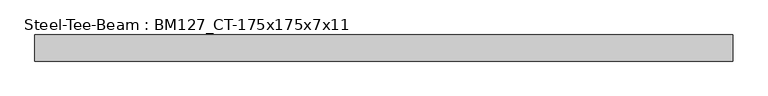
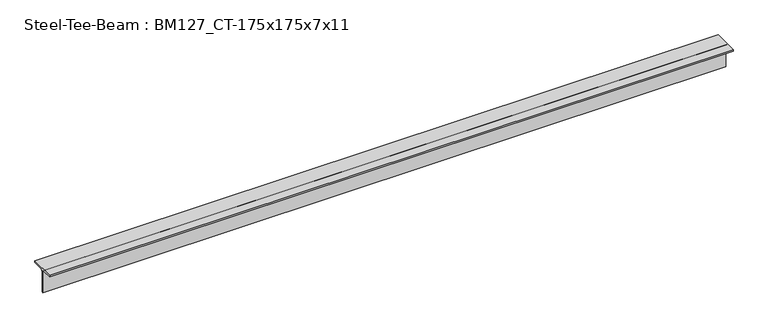
"""IFC4 building model written with IfcOpenShell, lengths in millimetres: beam geometry, Steel-Tee-Beam : BM127_CT-175x175x7x11."""

import ifcopenshell
import ifcopenshell.guid

model = None  # the IFC model being written
_history = None  # IfcOwnerHistory: only IFC2X3 demands one
_inside = {}  # id of a spatial element -> (the spatial element, [elements in it])
_under = {}  # id of a project, library or spatial element -> (it, [spatial elements below it])
_declared = {}  # id of a project -> (the project, [libraries it declares])
_typed = {}  # id of a type object -> (the type object, [elements of that type])
_made_of = {}  # id of a material, layer set ... -> (it, [elements and type objects made of it])


def new_model(schema):
    """Start an empty IFC model of exactly this schema.

    Asked for "IFC4X3", IfcOpenShell would pick the latest addendum, in which some entities
    have other attributes; the version numbers below select the first issue.
    IFC2X3 requires an IfcOwnerHistory on every rooted entity: one is made here for all.
    """
    global model, _history
    if schema == "IFC4X3":
        model = ifcopenshell.file(schema_version=(4, 3, 0, 0))
    else:
        model = ifcopenshell.file(schema=schema)
    _inside.clear()
    _under.clear()
    _declared.clear()
    _typed.clear()
    _made_of.clear()
    _history = None
    if model.schema == "IFC2X3":
        org = make("IfcOrganization", Name="unknown")
        user = make(
            "IfcPersonAndOrganization",
            ThePerson=make("IfcPerson", FamilyName="unknown"),
            TheOrganization=org,
        )
        app = make(
            "IfcApplication",
            ApplicationDeveloper=org,
            Version="unknown",
            ApplicationFullName="unknown",
            ApplicationIdentifier="unknown",
        )
        _history = make(
            "IfcOwnerHistory",
            OwningUser=user,
            OwningApplication=app,
            ChangeAction="ADDED",
            CreationDate=0,
        )
    return model


def make(cls, **values):
    """One entity of the class cls with the attributes given. An attribute that is None is left unset."""
    return model.create_entity(
        cls, **{name: value for name, value in values.items() if value is not None}
    )


def rooted(cls, **values):
    """An entity with a GlobalId (a new one), such as an element, a storey or a relation."""
    return make(cls, GlobalId=ifcopenshell.guid.new(), OwnerHistory=_history, **values)


def si_unit(unit_type, name, prefix=None):
    """IfcSIUnit, for example si_unit("LENGTHUNIT", "METRE", prefix="MILLI")."""
    return make("IfcSIUnit", UnitType=unit_type, Prefix=prefix, Name=name)


def assignment(units):
    """IfcUnitAssignment: the units of a project."""
    return None if units is None else make("IfcUnitAssignment", Units=units)


def point(xyz):
    """IfcCartesianPoint."""
    return None if xyz is None else make("IfcCartesianPoint", Coordinates=xyz)


def direction(xyz):
    """IfcDirection."""
    return None if xyz is None else make("IfcDirection", DirectionRatios=xyz)


def frame(location, z_axis=None, x_axis=None):
    """IfcAxis2Placement3D, a coordinate frame: its origin and axes. An axis left out is left unset."""
    return make(
        "IfcAxis2Placement3D",
        Location=point(location),
        Axis=direction(z_axis),
        RefDirection=direction(x_axis),
    )


def frame_2d(location, x_axis=None):
    """IfcAxis2Placement2D, a coordinate frame in the plane: its origin and x axis."""
    return make(
        "IfcAxis2Placement2D", Location=point(location), RefDirection=direction(x_axis)
    )


def origin():
    """The frame at (0, 0, 0) with its axes left unset."""
    return frame((0.0, 0.0, 0.0))


def place(relative_to, where):
    """IfcLocalPlacement: puts the frame where relative to a parent placement (None: the world)."""
    return make(
        "IfcLocalPlacement", PlacementRelTo=relative_to, RelativePlacement=where
    )


def context(
    kind, dimensions, precision=None, world=None, true_north=None, identifier=None
):
    """IfcGeometricRepresentationContext, for example the 3D "Model" context."""
    return make(
        "IfcGeometricRepresentationContext",
        ContextIdentifier=identifier,
        ContextType=kind,
        CoordinateSpaceDimension=dimensions,
        Precision=precision,
        WorldCoordinateSystem=world,
        TrueNorth=true_north,
    )


def project(units=None, contexts=None):
    """IfcProject with its units and contexts."""
    return rooted(
        "IfcProject",
        Name="project",
        RepresentationContexts=contexts,
        UnitsInContext=assignment(units),
    )


def spatial(cls, under=None, at=None, **own):
    """A site, building, storey or space (cls), placed at a placement, below another one or the project."""
    s = rooted(cls, ObjectPlacement=at, **own)
    if under is not None:
        _under.setdefault(under.id(), (under, []))[1].append(s)
    return s


def polyline(points):
    """IfcPolyline through the points."""
    return make("IfcPolyline", Points=[point(p) for p in points])


def circle_curve(where, radius):
    """IfcCircle in the frame where."""
    return make("IfcCircle", Position=where, Radius=radius)


def trimmed(basis, trim1, trim2, sense, master):
    """IfcTrimmedCurve: the piece of a basis curve between two trims."""
    return make(
        "IfcTrimmedCurve",
        BasisCurve=basis,
        Trim1=trim1,
        Trim2=trim2,
        SenseAgreement=sense,
        MasterRepresentation=master,
    )


def segment(curve, same_sense, transition):
    """IfcCompositeCurveSegment."""
    return make(
        "IfcCompositeCurveSegment",
        Transition=transition,
        SameSense=same_sense,
        ParentCurve=curve,
    )


def composite_curve(segments, self_intersect=None):
    """IfcCompositeCurve: segments joined end to end."""
    return make("IfcCompositeCurve", Segments=segments, SelfIntersect=self_intersect)


def outline(outer, holes=None, kind="AREA"):
    """IfcArbitraryClosedProfileDef: a profile drawn as a closed curve; with holes, ...WithVoids."""
    if holes is None:
        return make("IfcArbitraryClosedProfileDef", ProfileType=kind, OuterCurve=outer)
    return make(
        "IfcArbitraryProfileDefWithVoids",
        ProfileType=kind,
        OuterCurve=outer,
        InnerCurves=holes,
    )


def extrude(swept, where, along, depth):
    """IfcExtrudedAreaSolid: the profile swept, set in the frame where, extruded along a direction by depth."""
    return make(
        "IfcExtrudedAreaSolid",
        SweptArea=swept,
        Position=where,
        ExtrudedDirection=direction(along),
        Depth=depth,
    )


def shape(context_of_items, identifier, shape_type, items):
    """IfcShapeRepresentation: the items that make up one representation, for example the "Body"."""
    return make(
        "IfcShapeRepresentation",
        ContextOfItems=context_of_items,
        RepresentationIdentifier=identifier,
        RepresentationType=shape_type,
        Items=items,
    )


def source(mapping_origin, context_of_items, identifier, shape_type, items):
    """IfcRepresentationMap: a shape defined once, which mapped items show again and again."""
    return make(
        "IfcRepresentationMap",
        MappingOrigin=mapping_origin,
        MappedRepresentation=shape(context_of_items, identifier, shape_type, items),
    )


def transform(
    local_origin,
    x_axis=None,
    y_axis=None,
    z_axis=None,
    scale=None,
    scale2=None,
    scale3=None,
    uniform=True,
):
    """IfcCartesianTransformationOperator3D, or its non-uniform kind. x_axis, y_axis, z_axis: its Axis1, 2, 3."""
    if uniform:
        return make(
            "IfcCartesianTransformationOperator3D",
            Axis1=direction(x_axis),
            Axis2=direction(y_axis),
            LocalOrigin=point(local_origin),
            Scale=scale,
            Axis3=direction(z_axis),
        )
    return make(
        "IfcCartesianTransformationOperator3DnonUniform",
        Axis1=direction(x_axis),
        Axis2=direction(y_axis),
        LocalOrigin=point(local_origin),
        Scale=scale,
        Axis3=direction(z_axis),
        Scale2=scale2,
        Scale3=scale3,
    )


def mapped(mapping_source, mapping_target):
    """IfcMappedItem: shows the shape of a source again, moved by a transform."""
    return make(
        "IfcMappedItem", MappingSource=mapping_source, MappingTarget=mapping_target
    )


def made_of(thing, what):
    """Note that an element or type object is made of a material, layer set ...; save() writes the relation."""
    if what is not None:
        _made_of.setdefault(what.id(), (what, []))[1].append(thing)
    return thing


def element(
    cls,
    number,
    at=None,
    inside=None,
    cuts=None,
    type_object=None,
    material=None,
    context=None,
    identifier="Body",
    shape_type=None,
    held_by="IfcProductDefinitionShape",
    body=None,
    shapes=None,
    **own,
):
    """One element of the class cls, such as IfcWall. Its Tag is "e" and its number.

    at: its placement. inside: the storey or other place that contains it. cuts: it is an
    opening in that element (IfcRelVoidsElement). A single representation is given by context,
    identifier, shape_type and body (its items); several are given by shapes. held_by: the class
    of the entity that holds the representations. save() writes the other relations.
    """
    e = rooted(cls, Tag="e%d" % number, ObjectPlacement=at, **own)
    if body is not None:
        shapes = [shape(context, identifier, shape_type, body)]
    if shapes is not None:
        e.Representation = make(held_by, Representations=shapes)
    if inside is not None:
        _inside.setdefault(inside.id(), (inside, []))[1].append(e)
    if cuts is not None:
        rooted(
            "IfcRelVoidsElement", RelatingBuildingElement=cuts, RelatedOpeningElement=e
        )
    if type_object is not None:
        _typed.setdefault(type_object.id(), (type_object, []))[1].append(e)
    return made_of(e, material)


def aggregate(whole, parts):
    """IfcRelAggregates: a whole, such as a stair, and the parts it consists of."""
    return rooted("IfcRelAggregates", RelatingObject=whole, RelatedObjects=parts)


def save(model, path):
    """Write the relations noted so far, then the file.

    IfcRelAggregates (storeys below a building ...), IfcRelContainedInSpatialStructure (elements
    in a storey), IfcRelDefinesByType, IfcRelAssociatesMaterial and IfcRelDeclares: one each for
    every whole, place, type object, material and project.
    """
    for whole, parts in _under.values():
        aggregate(whole, parts)
    for where, things in _inside.values():
        rooted(
            "IfcRelContainedInSpatialStructure",
            RelatedElements=things,
            RelatingStructure=where,
        )
    for kind, things in _typed.values():
        rooted("IfcRelDefinesByType", RelatedObjects=things, RelatingType=kind)
    for what, things in _made_of.values():
        rooted("IfcRelAssociatesMaterial", RelatedObjects=things, RelatingMaterial=what)
    for by, libraries in _declared.values():
        rooted("IfcRelDeclares", RelatingContext=by, RelatedDefinitions=libraries)
    model.write(path)


def steel_tee_beam_bm127_ct_175x175x7x11_da8f831d(model_context):
    return source(origin(), model_context, "Body", "SweptSolid", [
        extrude(outline(composite_curve([segment(polyline([(87.5, 87.5), (87.5, 76.5), (17.5, 76.5)]), True, "CONTINUOUS"), segment(trimmed(circle_curve(frame_2d((17.5, 62.5)), 14.0), [point((17.5, 76.5))], [point((3.5, 62.5))], True, "CARTESIAN"), True, "CONTINUOUS"), segment(polyline([(3.5, 62.5), (3.5, -87.5), (-3.5, -87.5), (-3.5, 62.5)]), True, "CONTINUOUS"), segment(trimmed(circle_curve(frame_2d((-17.5, 62.5)), 14.0), [point((-3.5, 62.5))], [point((-17.5, 76.5))], True, "CARTESIAN"), True, "CONTINUOUS"), segment(polyline([(-17.5, 76.5), (-87.5, 76.5), (-87.5, 87.5), (87.5, 87.5)]), True, "CONTINUOUS")], self_intersect=False)), frame((-2365.2579713, 0.0, 0.0), z_axis=(1.0, 0.0, 0.0), x_axis=(0.0, 1.0, 0.0)), (0.0, 0.0, 1.0), 4669.2261367),
    ])


if __name__ == "__main__":
    model = new_model("IFC4")
    model_context = context("Model", 3, world=origin())
    ifc_project = project(units=[si_unit("LENGTHUNIT", "METRE", prefix="MILLI")], contexts=[model_context])
    site = spatial("IfcSite", under=ifc_project)
    building = spatial("IfcBuilding", under=site)
    placement = place(None, origin())
    steel_tee_beam_bm127_ct_175x175x7x11_shape = steel_tee_beam_bm127_ct_175x175x7x11_da8f831d(model_context)
    element("IfcBeam", 1, ObjectType="Steel-Tee-Beam : BM127_CT-175x175x7x11", at=placement, inside=building, context=model_context, shape_type="MappedRepresentation", body=[
        mapped(steel_tee_beam_bm127_ct_175x175x7x11_shape, transform((0.0, 0.0, 0.0), x_axis=(1.0, 0.0, 0.0), y_axis=(0.0, 1.0, 0.0), z_axis=(0.0, 0.0, 1.0))),
    ])
    save(model, "model.ifc")

# Revit data of these elements
# Type "Steel-Tee-Beam : BM127_CT-175x175x7x11"
#   Section Area = 31.57 cm²
#   Mass per Unit Length = 24.80 kg/m
#   Length [instance default] = 1524 mm
#   bf = 175 mm
#   d = 175 mm
#   k = 25 mm
#   kr = 14 mm
#   tf = 11 mm
#   tw = 7 mm
#   hec_material4 [instance default] = none
#   hec_material3 [instance default] = none
#   hec_material2 [instance default] = none
#   hec_material1 [instance default] = none
#   Structural Material [instance default] = Steel, 45-345
#   Assembly Code = ""
# Element 1 (IfcBeam, "Steel-Tee-Beam : BM127_CT-175x175x7x11")
#   hec_material3 = F01AC000-00002_Building/Shelter Fire Proofing Work_Intumescent Coating Type_1 hr. rating (UL 1709))
#   hec_material1 = S03AA029-00001_Main Steel Structure Erection Work_Shelter/Building_Light Steel
#   Structural Material = S01AA003-00001_Main Steel Structure Fabrication Work_Shelter/Building_Light Steel - Standard
#   Materials on its faces: "S01AA003-00001_Main Steel Structure Fabrication Work_Shelter/Building_Light Steel - Standard"
# Materials
#   "Steel, 45-345": class "Metal", colour RGB 189 187 185, transparency 0, Description = "Steel 345 MPa", Cost = 0
#   "S01AA003-00001_Main Steel Structure Fabrication Work_Shelter/Building_Light Steel - Standard": class "Metal", colour RGB 120 120 120, transparency 0, Comments = "(30KG/M>Weight)", Description = "Structural steel 50ksi", W00) Work Master Code = "S01AA003-00001", W01) Work Master_Lv1 = "Main Steel Structure Fabrication Work", W02) Work Master_Lv2 = "Shelter/Building", W03) Work Master_Spec.1 = "Light Steel - Standard (30KG/M>Weight)", Cost = 0
#   "F01AC000-00002_Building/Shelter Fire Proofing Work_Intumescent Coating Type_1 hr. rating (UL 1709))": class "Metal", colour RGB 255 128 128, transparency 0, Description = "Paint finished steel", W00) Work Master Code = "F01AC000-00002", W01) Work Master_Lv1 = "Building/Shelter Fire Proofing Work", W02) Work Master_Lv2 = "Intumescent Coating Type", W03) Work Master_Spec.1 = "1 hr. rating (UL 1709)", Cost = 0
#   "S03AA029-00001_Main Steel Structure Erection Work_Shelter/Building_Light Steel": class "Metal", colour RGB 120 120 120, transparency 0, Comments = "(30KG/M>Weight)", Description = "Structural steel 50ksi", W00) Work Master Code = "S03AA029-00001", W01) Work Master_Lv1 = "Main Steel Structure Erection Work", W02) Work Master_Lv2 = "Shelter/Building", W03) Work Master_Spec.1 = "Light Steel (30KG/M>Weight)", Cost = 0
